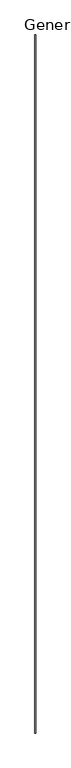
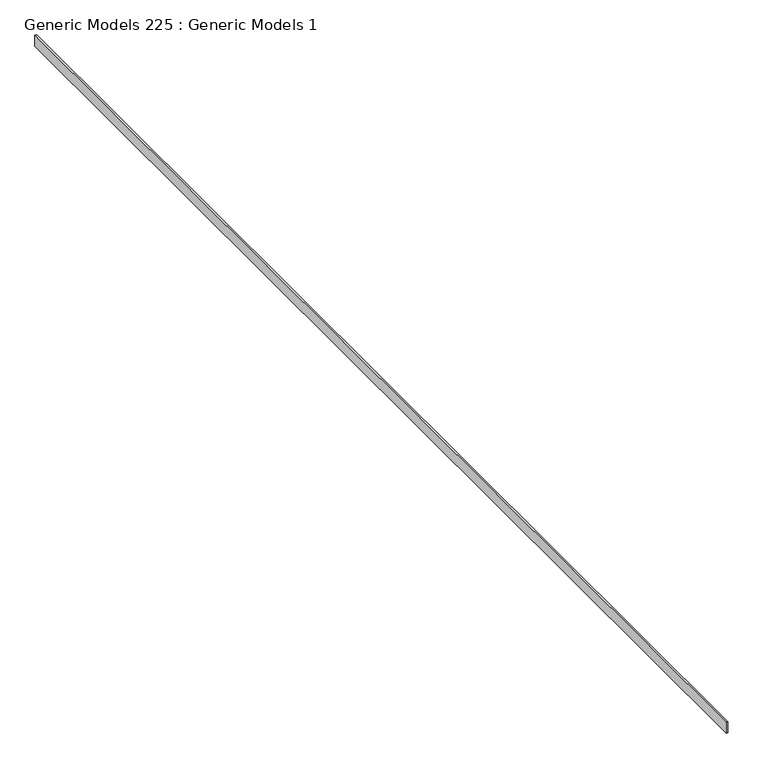
"""IFC4 building model written with IfcOpenShell, lengths in millimetres: proxy geometry, Generic Models 225 : Generic Models 1."""

from ifc_helpers import new_model, si_unit, frame, origin, place, context, project, spatial, polyline, outline, extrude, source, transform, mapped, element, save


def generic_models_225_generic_models_1_d58c226b(model_context):
    return source(origin(), model_context, "Body", "SweptSolid", [
        extrude(outline(polyline([(1795.013518, 306.6963299), (1783.901018, 306.6963299), (1783.901018, 8193.3963299), (1795.013518, 8193.3963299), (1795.013518, 306.6963299)])), frame((0.0, 0.0, 126236.6107803), z_axis=(0.0, 0.0, 1.0), x_axis=(1.0, 0.0, 0.0)), (0.0, 0.0, 1.0), 76.2),
    ])


if __name__ == "__main__":
    model = new_model("IFC4")
    model_context = context("Model", 3, world=origin())
    ifc_project = project(units=[si_unit("LENGTHUNIT", "METRE", prefix="MILLI")], contexts=[model_context])
    site = spatial("IfcSite", under=ifc_project)
    building = spatial("IfcBuilding", under=site)
    placement = place(None, origin())
    generic_models_225_generic_models_1_shape = generic_models_225_generic_models_1_d58c226b(model_context)
    element("IfcBuildingElementProxy", 1, Name="Generic Models 225 : Generic Models 1", ObjectType="Generic Models 225 : Generic Models 1", at=placement, inside=building, context=model_context, shape_type="MappedRepresentation", body=[
        mapped(generic_models_225_generic_models_1_shape, transform((0.0, 0.0, 0.0), x_axis=(1.0, 0.0, 0.0), y_axis=(0.0, 1.0, 0.0), z_axis=(0.0, 0.0, 1.0))),
    ])
    save(model, "model.ifc")

# Revit data of these elements
# Element 1 (IfcBuildingElementProxy, "Generic Models 225 : Generic Models 1")
#   Materials on its faces: "_SIDING VENT - COR-A-VENT - 7/16\" X 3\""
# Materials
#   "_SIDING VENT - COR-A-VENT - 7/16\" X 3\"": class "Generic", colour RGB 190 220 196, transparency 0, Cost = 0
